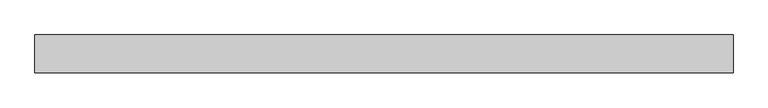
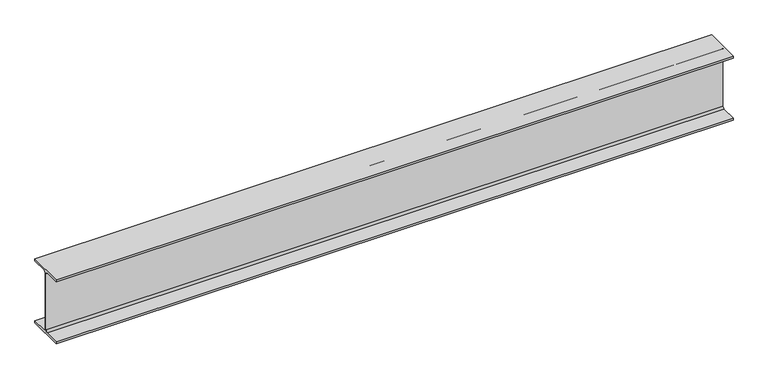
"""IFC4 building model written with IfcOpenShell, lengths in millimetres: beam geometry, Old_Steel Beam_H-KSD3502 : H_SB_ASB_H-200×200x8x12."""

from ifc_helpers import new_model, si_unit, point, frame, frame_2d, origin, place, context, project, spatial, polyline, circle_curve, trimmed, segment, composite_curve, outline, extrude, source, transform, mapped, element, save


def beam_620133c8(model_context):
    return source(origin(), model_context, "Body", "SweptSolid", [
        extrude(outline(composite_curve([segment(polyline([(82.5, -141.5), (82.5, -151.7), (-82.5, -151.7), (-82.5, -141.5), (-11.9, -141.5)]), True, "CONTINUOUS"), segment(trimmed(circle_curve(frame_2d((-11.9, -132.6)), 8.9), [point((-11.9, -141.5))], [point((-3.0, -132.6))], True, "CARTESIAN"), True, "CONTINUOUS"), segment(polyline([(-3.0, -132.6), (-3.0, 132.6)]), True, "CONTINUOUS"), segment(trimmed(circle_curve(frame_2d((-11.9, 132.6)), 8.9), [point((-3.0, 132.6))], [point((-11.9, 141.5))], True, "CARTESIAN"), True, "CONTINUOUS"), segment(polyline([(-11.9, 141.5), (-82.5, 141.5), (-82.5, 151.7), (82.5, 151.7), (82.5, 141.5), (11.9, 141.5)]), True, "CONTINUOUS"), segment(trimmed(circle_curve(frame_2d((11.9, 132.6)), 8.9), [point((11.9, 141.5))], [point((3.0, 132.6))], True, "CARTESIAN"), True, "CONTINUOUS"), segment(polyline([(3.0, 132.6), (3.0, -132.6)]), True, "CONTINUOUS"), segment(trimmed(circle_curve(frame_2d((11.9, -132.6)), 8.9), [point((3.0, -132.6))], [point((11.9, -141.5))], True, "CARTESIAN"), True, "CONTINUOUS"), segment(polyline([(11.9, -141.5), (82.5, -141.5)]), True, "CONTINUOUS")], self_intersect=False)), frame((-1325.5312133, 0.0, 0.0), z_axis=(1.0, 0.0, 0.0), x_axis=(0.0, 1.0, 0.0)), (0.0, 0.0, 1.0), 3025.785659),
    ])


if __name__ == "__main__":
    model = new_model("IFC4")
    model_context = context("Model", 3, world=origin())
    ifc_project = project(units=[si_unit("LENGTHUNIT", "METRE", prefix="MILLI")], contexts=[model_context])
    site = spatial("IfcSite", under=ifc_project)
    building = spatial("IfcBuilding", under=site)
    placement = place(None, origin())
    beam_shape = beam_620133c8(model_context)
    element("IfcBeam", 1, ObjectType="Old_Steel Beam_H-KSD3502 : H_SB_ASB_H-200×200x8x12", at=placement, inside=building, context=model_context, shape_type="MappedRepresentation", body=[
        mapped(beam_shape, transform((0.0, 0.0, 0.0), x_axis=(1.0, 0.0, 0.0), y_axis=(0.0, 1.0, 0.0), z_axis=(0.0, 0.0, 1.0))),
    ])
    save(model, "model.ifc")

# Revit data of these elements
# Type "Old_Steel Beam_H-KSD3502 : H_SB_ASB_H-200×200x8x12"
#   Width = 20.0 cm
#   Web Thickness = 0.8 cm
#   Web Fillet = 1.3 cm
#   Warping Constant = 141376.0 cm⁶
#   Torsional Moment of Inertia = 26.2485 cm⁴
#   Torsional Modulus = 1.0 cm³
#   Section Area = 63.53 cm²
#   Plastic Modulus weak axis = 244.0 cm³
#   Plastic Modulus strong axis = 525.0 cm³
#   Perimeter = 1.16 m²/m
#   Nominal Weight = 49.90 kgf/m
#   Moment of Inertia weak axis = 1600.00 cm⁴
#   Moment of Inertia strong axis = 4720.00 cm⁴
#   Height = 20.0 cm
#   Flange Thickness = 1.2 cm
#   Elastic Modulus weak axis = 160.0 cm³
#   Elastic Modulus strong axis = 472.0 cm³
#   Centroid Vertical = 10.0 cm
#   Centroid Horizontal = 10.0 cm
#   Length [instance default] = 1.5240 m
#   Structural Material [instance default] = Steel, 45-345
#   Assembly Code = ""
# Element 1 (IfcBeam, "Old_Steel Beam_H-KSD3502 : H_SB_ASB_H-200×200x8x12")
#   Structural Material = none
# Materials
#   "Steel, 45-345": class "Metal", colour RGB 189 187 185, transparency 0, Description = "Steel 345 MPa", Cost = 0
